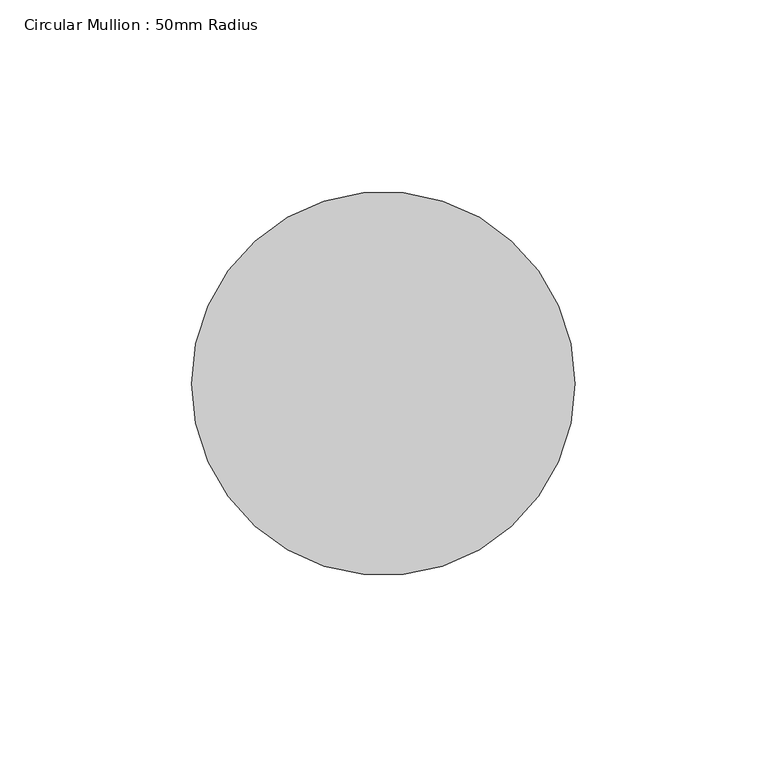
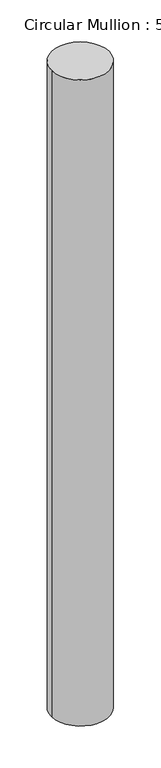
"""IFC4 building model written with IfcOpenShell, lengths in millimetres: member geometry, Circular Mullion : 50mm Radius."""

from ifc_helpers import new_model, si_unit, point, frame, origin, origin_2d, place, context, project, spatial, circle_curve, trimmed, segment, composite_curve, outline, extrude, source, transform, mapped, element, save


def circular_mullion_50mm_radius_6412449a(model_context):
    return source(origin(), model_context, "Body", "SweptSolid", [
        extrude(outline(composite_curve([segment(trimmed(circle_curve(origin_2d(), 50.0), [point((50.0, 0.0))], [point((-50.0, 0.0))], False, "CARTESIAN"), True, "CONTINUOUS"), segment(trimmed(circle_curve(origin_2d(), 50.0), [point((-50.0, 0.0))], [point((50.0, 0.0))], False, "CARTESIAN"), True, "CONTINUOUS")], self_intersect=False)), frame((0.0, 0.0, -1186.1855487), z_axis=(0.0, 0.0, 1.0), x_axis=(1.0, 0.0, 0.0)), (0.0, 0.0, 1.0), 1186.1855487),
    ])


if __name__ == "__main__":
    model = new_model("IFC4")
    model_context = context("Model", 3, world=origin())
    ifc_project = project(units=[si_unit("LENGTHUNIT", "METRE", prefix="MILLI")], contexts=[model_context])
    site = spatial("IfcSite", under=ifc_project)
    building = spatial("IfcBuilding", under=site)
    placement = place(None, origin())
    circular_mullion_50mm_radius_shape = circular_mullion_50mm_radius_6412449a(model_context)
    element("IfcMember", 1, ObjectType="Circular Mullion : 50mm Radius", at=placement, inside=building, context=model_context, shape_type="MappedRepresentation", body=[
        mapped(circular_mullion_50mm_radius_shape, transform((0.0, 0.0, 0.0), x_axis=(1.0, 0.0, 0.0), y_axis=(0.0, 1.0, 0.0), z_axis=(0.0, 0.0, 1.0))),
    ])
    save(model, "model.ifc")

# Revit data of these elements
# Type "Circular Mullion : 50mm Radius"
#   built-in parameter 1007350 = 0.164042 (stored number, unit not read)
# Element 1 (IfcMember, "Circular Mullion : 50mm Radius")
#   Materials on its faces: "Aluminium"
# Materials
#   "Aluminium": class "Metal", colour RGB 247 247 247, transparency 0, Description = "Aluminium 6061", Cost = 0
